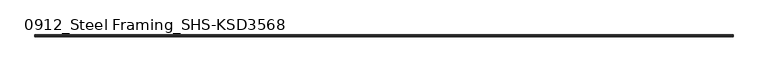
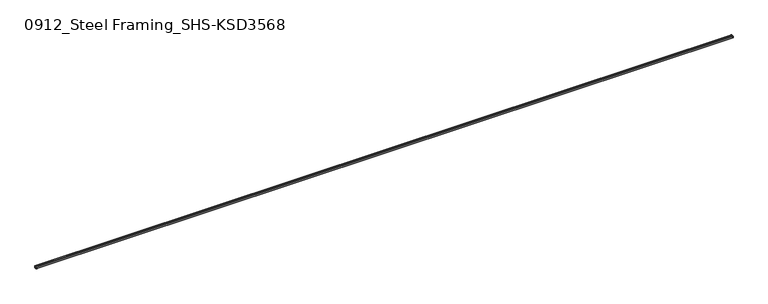
"""IFC4 building model written with IfcOpenShell, lengths in millimetres: beam geometry, 0912_Steel Framing_SHS-KSD3568 : H_SB_ASB_SHS-150x150x6."""

from ifc_helpers import new_model, si_unit, point, frame, frame_2d, origin, place, context, project, spatial, polyline, circle_curve, trimmed, segment, composite_curve, outline, extrude, source, transform, mapped, element, save


def beam_0912_steel_framing_shs_ksd3568_2f4f8f4d(model_context):
    return source(origin(), model_context, "Body", "SweptSolid", [
        extrude(outline(composite_curve([segment(polyline([(75.0, 63.0), (75.0, -63.0)]), True, "CONTINUOUS"), segment(trimmed(circle_curve(frame_2d((63.0, -63.0)), 12.0), [point((75.0, -63.0))], [point((63.0, -75.0))], False, "CARTESIAN"), True, "CONTINUOUS"), segment(polyline([(63.0, -75.0), (-63.0, -75.0)]), True, "CONTINUOUS"), segment(trimmed(circle_curve(frame_2d((-63.0, -63.0)), 12.0), [point((-63.0, -75.0))], [point((-75.0, -63.0))], False, "CARTESIAN"), True, "CONTINUOUS"), segment(polyline([(-75.0, -63.0), (-75.0, 63.0)]), True, "CONTINUOUS"), segment(trimmed(circle_curve(frame_2d((-63.0, 63.0)), 12.0), [point((-75.0, 63.0))], [point((-63.0, 75.0))], False, "CARTESIAN"), True, "CONTINUOUS"), segment(polyline([(-63.0, 75.0), (63.0, 75.0)]), True, "CONTINUOUS"), segment(trimmed(circle_curve(frame_2d((63.0, 63.0)), 12.0), [point((63.0, 75.0))], [point((75.0, 63.0))], False, "CARTESIAN"), True, "CONTINUOUS")], self_intersect=False), holes=[composite_curve([segment(trimmed(circle_curve(frame_2d((-63.0, 63.0)), 6.0), [point((-63.0, 69.0))], [point((-69.0, 63.0))], True, "CARTESIAN"), True, "CONTINUOUS"), segment(polyline([(-69.0, 63.0), (-69.0, -63.0)]), True, "CONTINUOUS"), segment(trimmed(circle_curve(frame_2d((-63.0, -63.0)), 6.0), [point((-69.0, -63.0))], [point((-63.0, -69.0))], True, "CARTESIAN"), True, "CONTINUOUS"), segment(polyline([(-63.0, -69.0), (63.0, -69.0)]), True, "CONTINUOUS"), segment(trimmed(circle_curve(frame_2d((63.0, -63.0)), 6.0), [point((63.0, -69.0))], [point((69.0, -63.0))], True, "CARTESIAN"), True, "CONTINUOUS"), segment(polyline([(69.0, -63.0), (69.0, 63.0)]), True, "CONTINUOUS"), segment(trimmed(circle_curve(frame_2d((63.0, 63.0)), 6.0), [point((69.0, 63.0))], [point((63.0, 69.0))], True, "CARTESIAN"), True, "CONTINUOUS"), segment(polyline([(63.0, 69.0), (-63.0, 69.0)]), True, "CONTINUOUS")], self_intersect=False)]), frame((-25622.5, 0.0, 0.0), z_axis=(1.0, 0.0, 0.0), x_axis=(0.0, 1.0, 0.0)), (0.0, 0.0, 1.0), 51245.0),
    ])


if __name__ == "__main__":
    model = new_model("IFC4")
    model_context = context("Model", 3, world=origin())
    ifc_project = project(units=[si_unit("LENGTHUNIT", "METRE", prefix="MILLI")], contexts=[model_context])
    site = spatial("IfcSite", under=ifc_project)
    building = spatial("IfcBuilding", under=site)
    placement = place(None, origin())
    beam_0912_steel_framing_shs_ksd3568_shape = beam_0912_steel_framing_shs_ksd3568_2f4f8f4d(model_context)
    element("IfcBeam", 1, ObjectType="0912_Steel Framing_SHS-KSD3568 : H_SB_ASB_SHS-150x150x6", at=placement, inside=building, context=model_context, shape_type="MappedRepresentation", body=[
        mapped(beam_0912_steel_framing_shs_ksd3568_shape, transform((0.0, 0.0, 0.0), x_axis=(1.0, 0.0, 0.0), y_axis=(0.0, 1.0, 0.0), z_axis=(0.0, 0.0, 1.0))),
    ])
    save(model, "model.ifc")

# Revit data of these elements
# Type "0912_Steel Framing_SHS-KSD3568 : H_SB_ASB_SHS-150x150x6"
#   H_WM Code_1 = "S01AA002-00001 | Main Steel Structure Fabrication Work | Shelter/Building | Medium Steel - Standard (90KG/M>Weight≥30KG/M) | Material: (   )"
#   H_WM Code_2 = "S03AA028-00001 | Main Steel Structure Erection Work | Shelter/Building | Medium Steel (90KG/M>Weight≥30KG/M) | Material: (   )"
#   H_WM Code_3 = "S01AA010-00001 | Main Steel Structure Fabrication Work | Shelter/Building | Steel Painting/Coating | for Non-Fireproofed Steel Surface, Surface Preparation, Primer, Second & Final Coat | Material: (   )"
#   H_Q'ty Cal Type Tag = "SB-Q2"
#   Perimeter = 0.60 m²/m
#   Nominal Weight = 26.40 kgf/m
#   Length [instance default] = 1.0000 m
#   b = 0.1500 m
#   h = 0.1500 m
#   tr = 0.0120 m
#   t = 0.0060 m
#   A = 28.36 m²
#   Structural Material [instance default] = Steel, 45-345
# Element 1 (IfcBeam, "0912_Steel Framing_SHS-KSD3568 : H_SB_ASB_SHS-150x150x6")
#   Structural Material = none
# Materials
#   "Steel, 45-345": class "Metal", colour RGB 189 187 185, transparency 0, Description = "Steel 345 MPa", Cost = 0
